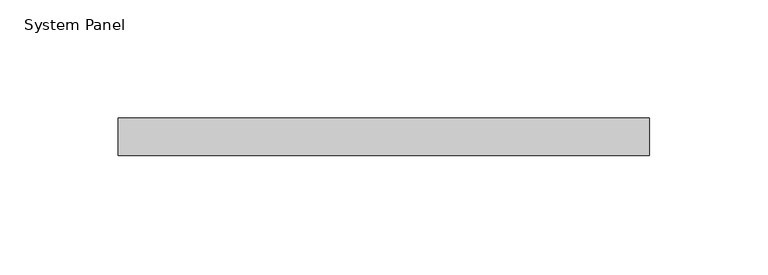
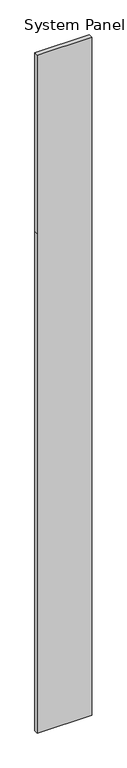
"""IFC4 building model written with IfcOpenShell, lengths in millimetres: plate geometry, System Panel : 로이복층유리_16."""

import ifcopenshell
import ifcopenshell.guid

model = None  # the IFC model being written
_history = None  # IfcOwnerHistory: only IFC2X3 demands one
_inside = {}  # id of a spatial element -> (the spatial element, [elements in it])
_under = {}  # id of a project, library or spatial element -> (it, [spatial elements below it])
_declared = {}  # id of a project -> (the project, [libraries it declares])
_typed = {}  # id of a type object -> (the type object, [elements of that type])
_made_of = {}  # id of a material, layer set ... -> (it, [elements and type objects made of it])


def new_model(schema):
    """Start an empty IFC model of exactly this schema.

    Asked for "IFC4X3", IfcOpenShell would pick the latest addendum, in which some entities
    have other attributes; the version numbers below select the first issue.
    IFC2X3 requires an IfcOwnerHistory on every rooted entity: one is made here for all.
    """
    global model, _history
    if schema == "IFC4X3":
        model = ifcopenshell.file(schema_version=(4, 3, 0, 0))
    else:
        model = ifcopenshell.file(schema=schema)
    _inside.clear()
    _under.clear()
    _declared.clear()
    _typed.clear()
    _made_of.clear()
    _history = None
    if model.schema == "IFC2X3":
        org = make("IfcOrganization", Name="unknown")
        user = make(
            "IfcPersonAndOrganization",
            ThePerson=make("IfcPerson", FamilyName="unknown"),
            TheOrganization=org,
        )
        app = make(
            "IfcApplication",
            ApplicationDeveloper=org,
            Version="unknown",
            ApplicationFullName="unknown",
            ApplicationIdentifier="unknown",
        )
        _history = make(
            "IfcOwnerHistory",
            OwningUser=user,
            OwningApplication=app,
            ChangeAction="ADDED",
            CreationDate=0,
        )
    return model


def make(cls, **values):
    """One entity of the class cls with the attributes given. An attribute that is None is left unset."""
    return model.create_entity(
        cls, **{name: value for name, value in values.items() if value is not None}
    )


def rooted(cls, **values):
    """An entity with a GlobalId (a new one), such as an element, a storey or a relation."""
    return make(cls, GlobalId=ifcopenshell.guid.new(), OwnerHistory=_history, **values)


def si_unit(unit_type, name, prefix=None):
    """IfcSIUnit, for example si_unit("LENGTHUNIT", "METRE", prefix="MILLI")."""
    return make("IfcSIUnit", UnitType=unit_type, Prefix=prefix, Name=name)


def assignment(units):
    """IfcUnitAssignment: the units of a project."""
    return None if units is None else make("IfcUnitAssignment", Units=units)


def point(xyz):
    """IfcCartesianPoint."""
    return None if xyz is None else make("IfcCartesianPoint", Coordinates=xyz)


def direction(xyz):
    """IfcDirection."""
    return None if xyz is None else make("IfcDirection", DirectionRatios=xyz)


def frame(location, z_axis=None, x_axis=None):
    """IfcAxis2Placement3D, a coordinate frame: its origin and axes. An axis left out is left unset."""
    return make(
        "IfcAxis2Placement3D",
        Location=point(location),
        Axis=direction(z_axis),
        RefDirection=direction(x_axis),
    )


def origin():
    """The frame at (0, 0, 0) with its axes left unset."""
    return frame((0.0, 0.0, 0.0))


def place(relative_to, where):
    """IfcLocalPlacement: puts the frame where relative to a parent placement (None: the world)."""
    return make(
        "IfcLocalPlacement", PlacementRelTo=relative_to, RelativePlacement=where
    )


def context(
    kind, dimensions, precision=None, world=None, true_north=None, identifier=None
):
    """IfcGeometricRepresentationContext, for example the 3D "Model" context."""
    return make(
        "IfcGeometricRepresentationContext",
        ContextIdentifier=identifier,
        ContextType=kind,
        CoordinateSpaceDimension=dimensions,
        Precision=precision,
        WorldCoordinateSystem=world,
        TrueNorth=true_north,
    )


def project(units=None, contexts=None):
    """IfcProject with its units and contexts."""
    return rooted(
        "IfcProject",
        Name="project",
        RepresentationContexts=contexts,
        UnitsInContext=assignment(units),
    )


def spatial(cls, under=None, at=None, **own):
    """A site, building, storey or space (cls), placed at a placement, below another one or the project."""
    s = rooted(cls, ObjectPlacement=at, **own)
    if under is not None:
        _under.setdefault(under.id(), (under, []))[1].append(s)
    return s


def polyline(points):
    """IfcPolyline through the points."""
    return make("IfcPolyline", Points=[point(p) for p in points])


def outline(outer, holes=None, kind="AREA"):
    """IfcArbitraryClosedProfileDef: a profile drawn as a closed curve; with holes, ...WithVoids."""
    if holes is None:
        return make("IfcArbitraryClosedProfileDef", ProfileType=kind, OuterCurve=outer)
    return make(
        "IfcArbitraryProfileDefWithVoids",
        ProfileType=kind,
        OuterCurve=outer,
        InnerCurves=holes,
    )


def extrude(swept, where, along, depth):
    """IfcExtrudedAreaSolid: the profile swept, set in the frame where, extruded along a direction by depth."""
    return make(
        "IfcExtrudedAreaSolid",
        SweptArea=swept,
        Position=where,
        ExtrudedDirection=direction(along),
        Depth=depth,
    )


def shape(context_of_items, identifier, shape_type, items):
    """IfcShapeRepresentation: the items that make up one representation, for example the "Body"."""
    return make(
        "IfcShapeRepresentation",
        ContextOfItems=context_of_items,
        RepresentationIdentifier=identifier,
        RepresentationType=shape_type,
        Items=items,
    )


def source(mapping_origin, context_of_items, identifier, shape_type, items):
    """IfcRepresentationMap: a shape defined once, which mapped items show again and again."""
    return make(
        "IfcRepresentationMap",
        MappingOrigin=mapping_origin,
        MappedRepresentation=shape(context_of_items, identifier, shape_type, items),
    )


def transform(
    local_origin,
    x_axis=None,
    y_axis=None,
    z_axis=None,
    scale=None,
    scale2=None,
    scale3=None,
    uniform=True,
):
    """IfcCartesianTransformationOperator3D, or its non-uniform kind. x_axis, y_axis, z_axis: its Axis1, 2, 3."""
    if uniform:
        return make(
            "IfcCartesianTransformationOperator3D",
            Axis1=direction(x_axis),
            Axis2=direction(y_axis),
            LocalOrigin=point(local_origin),
            Scale=scale,
            Axis3=direction(z_axis),
        )
    return make(
        "IfcCartesianTransformationOperator3DnonUniform",
        Axis1=direction(x_axis),
        Axis2=direction(y_axis),
        LocalOrigin=point(local_origin),
        Scale=scale,
        Axis3=direction(z_axis),
        Scale2=scale2,
        Scale3=scale3,
    )


def mapped(mapping_source, mapping_target):
    """IfcMappedItem: shows the shape of a source again, moved by a transform."""
    return make(
        "IfcMappedItem", MappingSource=mapping_source, MappingTarget=mapping_target
    )


def made_of(thing, what):
    """Note that an element or type object is made of a material, layer set ...; save() writes the relation."""
    if what is not None:
        _made_of.setdefault(what.id(), (what, []))[1].append(thing)
    return thing


def element(
    cls,
    number,
    at=None,
    inside=None,
    cuts=None,
    type_object=None,
    material=None,
    context=None,
    identifier="Body",
    shape_type=None,
    held_by="IfcProductDefinitionShape",
    body=None,
    shapes=None,
    **own,
):
    """One element of the class cls, such as IfcWall. Its Tag is "e" and its number.

    at: its placement. inside: the storey or other place that contains it. cuts: it is an
    opening in that element (IfcRelVoidsElement). A single representation is given by context,
    identifier, shape_type and body (its items); several are given by shapes. held_by: the class
    of the entity that holds the representations. save() writes the other relations.
    """
    e = rooted(cls, Tag="e%d" % number, ObjectPlacement=at, **own)
    if body is not None:
        shapes = [shape(context, identifier, shape_type, body)]
    if shapes is not None:
        e.Representation = make(held_by, Representations=shapes)
    if inside is not None:
        _inside.setdefault(inside.id(), (inside, []))[1].append(e)
    if cuts is not None:
        rooted(
            "IfcRelVoidsElement", RelatingBuildingElement=cuts, RelatedOpeningElement=e
        )
    if type_object is not None:
        _typed.setdefault(type_object.id(), (type_object, []))[1].append(e)
    return made_of(e, material)


def aggregate(whole, parts):
    """IfcRelAggregates: a whole, such as a stair, and the parts it consists of."""
    return rooted("IfcRelAggregates", RelatingObject=whole, RelatedObjects=parts)


def save(model, path):
    """Write the relations noted so far, then the file.

    IfcRelAggregates (storeys below a building ...), IfcRelContainedInSpatialStructure (elements
    in a storey), IfcRelDefinesByType, IfcRelAssociatesMaterial and IfcRelDeclares: one each for
    every whole, place, type object, material and project.
    """
    for whole, parts in _under.values():
        aggregate(whole, parts)
    for where, things in _inside.values():
        rooted(
            "IfcRelContainedInSpatialStructure",
            RelatedElements=things,
            RelatingStructure=where,
        )
    for kind, things in _typed.values():
        rooted("IfcRelDefinesByType", RelatedObjects=things, RelatingType=kind)
    for what, things in _made_of.values():
        rooted("IfcRelAssociatesMaterial", RelatedObjects=things, RelatingMaterial=what)
    for by, libraries in _declared.values():
        rooted("IfcRelDeclares", RelatingContext=by, RelatedDefinitions=libraries)
    model.write(path)


def system_panel_827ed390(model_context):
    return source(origin(), model_context, "Body", "SweptSolid", [
        extrude(outline(polyline([(0.0, -112.5), (0.0, 112.5), (2177.5, 112.5), (2955.0, 112.5), (2955.0, -112.5), (2177.5, -112.5), (0.0, -112.5)])), frame((0.0, -8.0, 0.0), z_axis=(0.0, 1.0, 0.0), x_axis=(0.0, 0.0, 1.0)), (0.0, 0.0, 1.0), 16.0),
    ])


if __name__ == "__main__":
    model = new_model("IFC4")
    model_context = context("Model", 3, world=origin())
    ifc_project = project(units=[si_unit("LENGTHUNIT", "METRE", prefix="MILLI")], contexts=[model_context])
    site = spatial("IfcSite", under=ifc_project)
    building = spatial("IfcBuilding", under=site)
    placement = place(None, origin())
    system_panel_shape = system_panel_827ed390(model_context)
    element("IfcPlate", 1, ObjectType="System Panel : 로이복층유리_16", at=placement, inside=building, context=model_context, shape_type="MappedRepresentation", body=[
        mapped(system_panel_shape, transform((0.0, 0.0, 0.0), x_axis=(1.0, 0.0, 0.0), y_axis=(0.0, 1.0, 0.0), z_axis=(0.0, 0.0, 1.0))),
    ])
    save(model, "model.ifc")

# Revit data of these elements
# Element 1 (IfcPlate, "System Panel : 로이복층유리_16")
#   Materials on its faces: "00_Glass_Glass"
# Materials
#   "00_Glass_Glass": class "Glass", colour RGB 218 227 224, transparency 0.85, Description = "Glass", Cost = 0, Image = none
